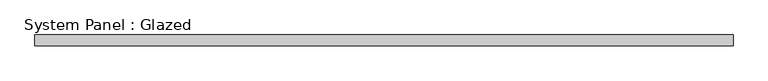
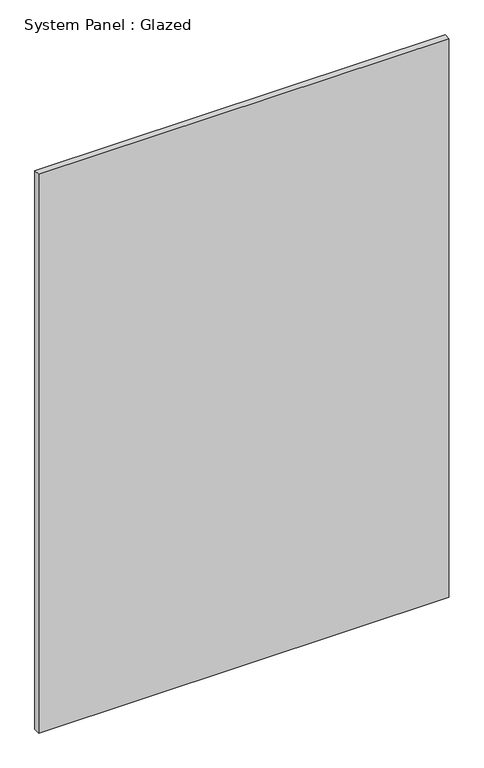
"""IFC4 building model written with IfcOpenShell, lengths in millimetres: plate geometry, System Panel : Glazed."""

from ifc_helpers import new_model, si_unit, origin, origin_with_axes, place, context, project, spatial, polyline, outline, extrude, source, transform, mapped, element, save


def system_panel_glazed_3f56aabd(model_context):
    return source(origin(), model_context, "Body", "SweptSolid", [
        extrude(outline(polyline([(807.5, 24.5), (-807.5, 24.5), (-807.5, 49.5), (807.5, 49.5), (807.5, 24.5)])), origin_with_axes(), (0.0, 0.0, 1.0), 2325.0),
    ])


if __name__ == "__main__":
    model = new_model("IFC4")
    model_context = context("Model", 3, world=origin())
    ifc_project = project(units=[si_unit("LENGTHUNIT", "METRE", prefix="MILLI")], contexts=[model_context])
    site = spatial("IfcSite", under=ifc_project)
    building = spatial("IfcBuilding", under=site)
    placement = place(None, origin())
    system_panel_glazed_shape = system_panel_glazed_3f56aabd(model_context)
    element("IfcPlate", 1, ObjectType="System Panel : Glazed", at=placement, inside=building, context=model_context, shape_type="MappedRepresentation", body=[
        mapped(system_panel_glazed_shape, transform((0.0, 0.0, 0.0), x_axis=(1.0, 0.0, 0.0), y_axis=(0.0, 1.0, 0.0), z_axis=(0.0, 0.0, 1.0))),
    ])
    save(model, "model.ifc")

# Revit data of these elements
# Element 1 (IfcPlate, "System Panel : Glazed")
#   Materials on its faces: "Glass"
# Materials
#   "Glass": class "Glass", colour RGB 0 128 192, transparency 0.9
